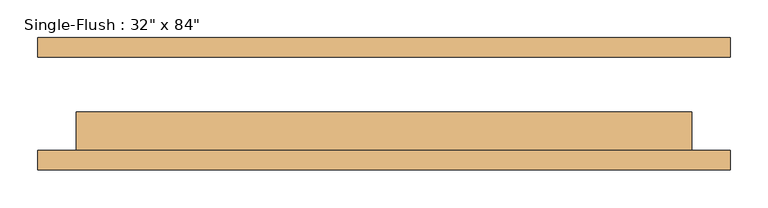
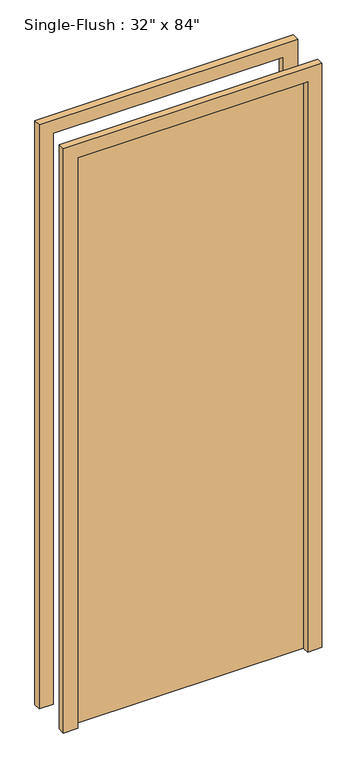
"""IFC4 building model written with IfcOpenShell, lengths in millimetres: door geometry."""

from ifc_helpers import new_model, si_unit, frame, origin, origin_with_axes, place, context, project, spatial, polyline, outline, extrude, source, transform, mapped, element, save


def door_0053c20e(model_context):
    return source(origin(), model_context, "Body", "SweptSolid", [
        extrude(outline(polyline([(2184.4, -457.2), (0.0, -457.2), (0.0, -406.4), (2133.6, -406.4), (2133.6, 406.4), (0.0, 406.4), (0.0, 457.2), (2184.4, 457.2), (2184.4, -457.2)])), frame((0.0, -87.3125, 0.0), z_axis=(0.0, 1.0, 0.0), x_axis=(0.0, 0.0, 1.0)), (0.0, 0.0, 1.0), 25.4),
        extrude(outline(polyline([(2184.4, 457.2), (2184.4, -457.2), (0.0, -457.2), (0.0, -406.4), (2133.6, -406.4), (2133.6, 406.4), (0.0, 406.4), (0.0, 457.2), (2184.4, 457.2)])), frame((0.0, 61.9125, 0.0), z_axis=(0.0, 1.0, 0.0), x_axis=(0.0, 0.0, 1.0)), (0.0, 0.0, 1.0), 25.4),
        extrude(outline(polyline([(406.4, -11.1125), (406.4, -61.9125), (-406.4, -61.9125), (-406.4, -11.1125), (406.4, -11.1125)])), origin_with_axes(), (0.0, 0.0, 1.0), 2133.6),
    ])


if __name__ == "__main__":
    model = new_model("IFC4")
    model_context = context("Model", 3, world=origin())
    ifc_project = project(units=[si_unit("LENGTHUNIT", "METRE", prefix="MILLI")], contexts=[model_context])
    site = spatial("IfcSite", under=ifc_project)
    building = spatial("IfcBuilding", under=site)
    placement = place(None, origin())
    door_shape = door_0053c20e(model_context)
    element("IfcDoor", 1, ObjectType="Single-Flush : 32\" x 84\"", at=placement, inside=building, context=model_context, shape_type="MappedRepresentation", body=[
        mapped(door_shape, transform((0.0, 0.0, 0.0), x_axis=(1.0, 0.0, 0.0), y_axis=(0.0, 1.0, 0.0), z_axis=(0.0, 0.0, 1.0))),
    ])
    save(model, "model.ifc")

# Revit data of these elements
# Project information
#   Project Issue Date = "07/20/2015"
#   Project Status = "Project Status"
#   Client Name = "Xcel"
#   Project Address = "Enter address here"
#   Project Name = "Sports Complex"
#   Project Number = "Project Number"
# Type "Single-Flush : 32\" x 84\""
#   Type Mark = "10"
#   Construction Type Id = "MDOOR"
#   Assembly Code = "C1020"
#   Analytic Construction = "Metal"
#   Thickness = 0' - 2"
#   Heat Transfer Coefficient (U) = 3.7021 W/(m²·K)
#   Height = 7' - 0"
#   Trim Projection Ext = 0' - 1"
#   Trim Projection Int = 0' - 1"
#   Trim Width = 0' - 2"
#   Width = 2' - 8"
#   Door Material = Door - Panel
#   Frame Material = Door - Frame
#   Visual Light Transmittance = 0
#   Solar Heat Gain Coefficient = 0
#   Function = (empty or 0)
#   Wall Closure = (empty or 0)
# Element 1 (IfcDoor, "Single-Flush : 32\" x 84\"")
#   Materials on its faces: "Door - Frame", "Door - Panel"
# Materials
#   "Door - Panel": class "Wood", colour RGB 212 179 113, transparency 0, Cost = 0
#   "Door - Frame": class "Miscellaneous", colour RGB 65 65 65, transparency 0, Cost = 0
